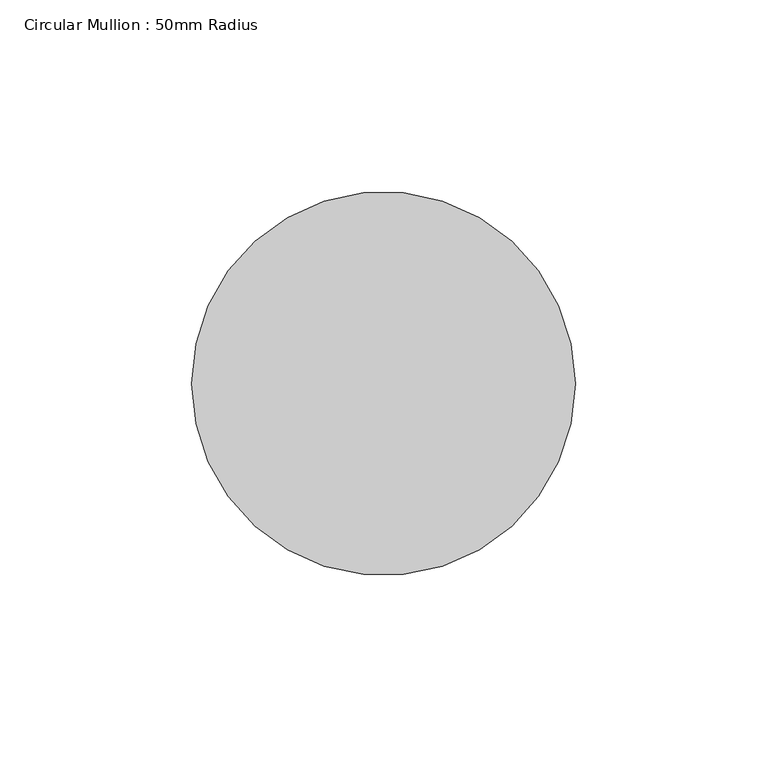
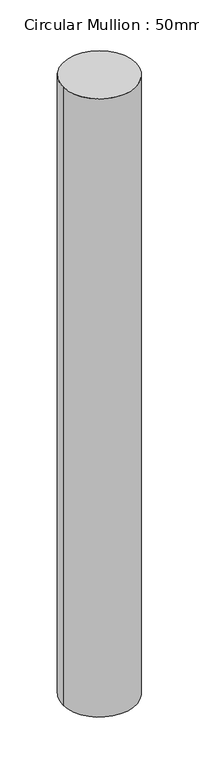
"""IFC4 building model written with IfcOpenShell, lengths in millimetres: member geometry, Circular Mullion : 50mm Radius."""

from ifc_helpers import new_model, si_unit, point, frame, origin, origin_2d, place, context, project, spatial, circle_curve, trimmed, segment, composite_curve, outline, extrude, source, transform, mapped, element, save


def circular_mullion_50mm_radius_60edfac6(model_context):
    return source(origin(), model_context, "Body", "SweptSolid", [
        extrude(outline(composite_curve([segment(trimmed(circle_curve(origin_2d(), 50.0), [point((50.0, 0.0))], [point((-50.0, 0.0))], False, "CARTESIAN"), True, "CONTINUOUS"), segment(trimmed(circle_curve(origin_2d(), 50.0), [point((-50.0, 0.0))], [point((50.0, 0.0))], False, "CARTESIAN"), True, "CONTINUOUS")], self_intersect=False)), frame((0.0, 0.0, -898.1569839), z_axis=(0.0, 0.0, 1.0), x_axis=(1.0, 0.0, 0.0)), (0.0, 0.0, 1.0), 898.1569839),
    ])


if __name__ == "__main__":
    model = new_model("IFC4")
    model_context = context("Model", 3, world=origin())
    ifc_project = project(units=[si_unit("LENGTHUNIT", "METRE", prefix="MILLI")], contexts=[model_context])
    site = spatial("IfcSite", under=ifc_project)
    building = spatial("IfcBuilding", under=site)
    placement = place(None, origin())
    circular_mullion_50mm_radius_shape = circular_mullion_50mm_radius_60edfac6(model_context)
    element("IfcMember", 1, ObjectType="Circular Mullion : 50mm Radius", at=placement, inside=building, context=model_context, shape_type="MappedRepresentation", body=[
        mapped(circular_mullion_50mm_radius_shape, transform((0.0, 0.0, 0.0), x_axis=(1.0, 0.0, 0.0), y_axis=(0.0, 1.0, 0.0), z_axis=(0.0, 0.0, 1.0))),
    ])
    save(model, "model.ifc")

# Revit data of these elements
# Type "Circular Mullion : 50mm Radius"
#   built-in parameter 1007350 = 0.164042 (stored number, unit not read)
# Element 1 (IfcMember, "Circular Mullion : 50mm Radius")
#   Materials on its faces: "Aluminium"
# Materials
#   "Aluminium": class "Metal", colour RGB 247 247 247, transparency 0, Description = "Aluminium 6061", Cost = 0
